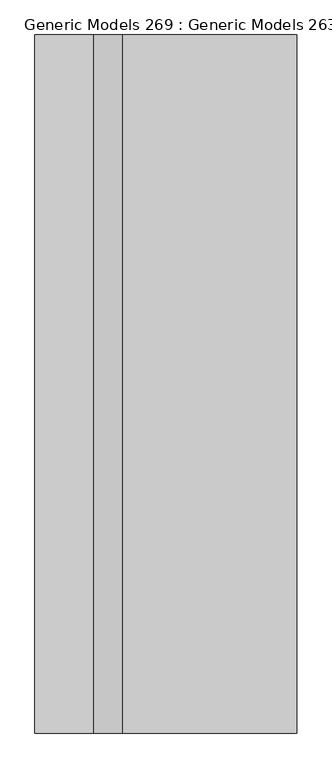
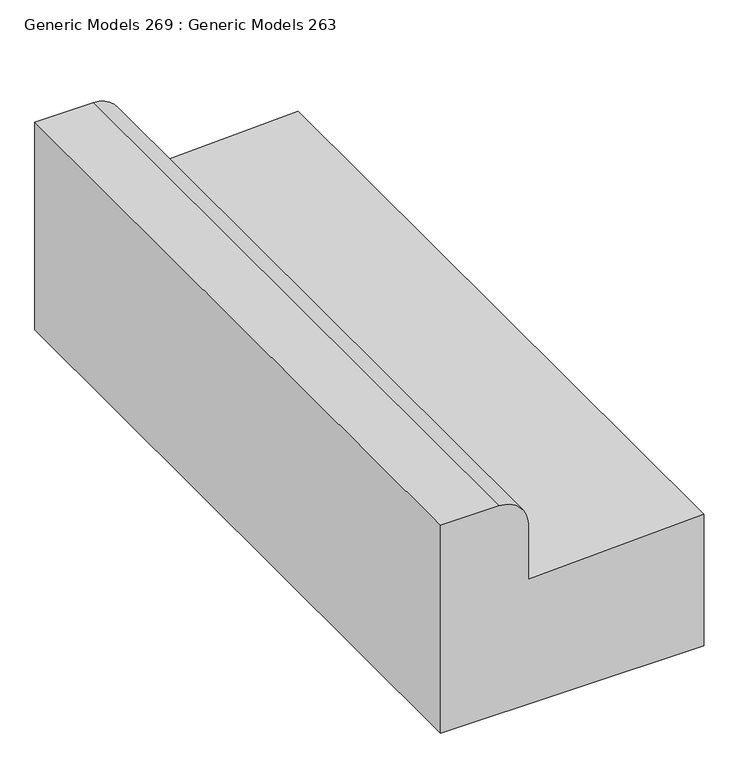
"""IFC4 building model written with IfcOpenShell, lengths in millimetres: proxy geometry, Generic Models 269 : Generic Models 263."""

from ifc_helpers import new_model, si_unit, point, frame, frame_2d, origin, place, context, project, spatial, polyline, circle_curve, trimmed, segment, composite_curve, outline, extrude, source, transform, mapped, element, save


def generic_models_269_generic_models_263_66db3b1b(model_context):
    return source(origin(), model_context, "Body", "SweptSolid", [
        extrude(outline(composite_curve([segment(polyline([(0.0, 60591.9797726), (0.0, 60490.3797726), (-381.0, 60490.3797726), (-381.0, 60947.5797726), (-139.7, 60947.5797726), (-152.4, 60642.7797726), (-50.8, 60642.7797726)]), True, "CONTINUOUS"), segment(trimmed(circle_curve(frame_2d((-50.8, 60591.9797726)), 50.8), [point((-50.8, 60642.7797726))], [point((0.0, 60591.9797726))], False, "CARTESIAN"), True, "CONTINUOUS")], self_intersect=False)), frame((0.0, -94.4486541, 0.0), z_axis=(0.0, 1.0, 0.0), x_axis=(0.0, 0.0, 1.0)), (0.0, 0.0, 1.0), 1219.2),
    ])


if __name__ == "__main__":
    model = new_model("IFC4")
    model_context = context("Model", 3, world=origin())
    ifc_project = project(units=[si_unit("LENGTHUNIT", "METRE", prefix="MILLI")], contexts=[model_context])
    site = spatial("IfcSite", under=ifc_project)
    building = spatial("IfcBuilding", under=site)
    placement = place(None, origin())
    generic_models_269_generic_models_263_shape = generic_models_269_generic_models_263_66db3b1b(model_context)
    element("IfcBuildingElementProxy", 1, Name="Generic Models 269 : Generic Models 263", ObjectType="Generic Models 269 : Generic Models 263", at=placement, inside=building, context=model_context, shape_type="MappedRepresentation", body=[
        mapped(generic_models_269_generic_models_263_shape, transform((0.0, 0.0, 0.0), x_axis=(1.0, 0.0, 0.0), y_axis=(0.0, 1.0, 0.0), z_axis=(0.0, 0.0, 1.0))),
    ])
    save(model, "model.ifc")

# Revit data of these elements
# Element 1 (IfcBuildingElementProxy, "Generic Models 269 : Generic Models 263")
#   Materials on its faces: "CONCRETE CURB"
# Materials
#   "CONCRETE CURB": class "Concrete", colour RGB 191 191 191, transparency 0, Description = "Cast-in-place concrete", Cost = 0
